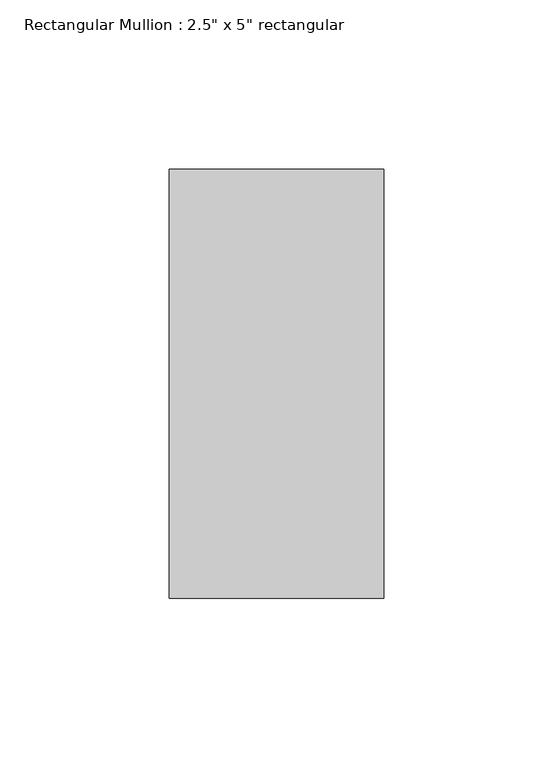
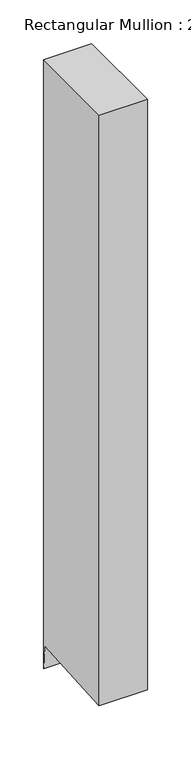
"""IFC4 building model written with IfcOpenShell, lengths in millimetres: member geometry."""

from ifc_helpers import new_model, si_unit, frame, origin, place, context, project, spatial, polyline, outline, extrude, source, transform, mapped, element, save


def member_bfce15ef(model_context):
    return source(origin(), model_context, "Body", "SweptSolid", [
        extrude(outline(polyline([(-63.5, 0.0), (63.5, 0.0), (63.5, -848.9346233), (61.4149606, -815.2837802), (-63.5, -823.0236342), (-63.5, 0.0)])), frame((-63.5, 0.0, 0.0), z_axis=(1.0, 0.0, 0.0), x_axis=(0.0, 1.0, 0.0)), (0.0, 0.0, 1.0), 63.5),
    ])


if __name__ == "__main__":
    model = new_model("IFC4")
    model_context = context("Model", 3, world=origin())
    ifc_project = project(units=[si_unit("LENGTHUNIT", "METRE", prefix="MILLI")], contexts=[model_context])
    site = spatial("IfcSite", under=ifc_project)
    building = spatial("IfcBuilding", under=site)
    placement = place(None, origin())
    member_shape = member_bfce15ef(model_context)
    element("IfcMember", 1, ObjectType="Rectangular Mullion : 2.5\" x 5\" rectangular", at=placement, inside=building, context=model_context, shape_type="MappedRepresentation", body=[
        mapped(member_shape, transform((0.0, 0.0, 0.0), x_axis=(1.0, 0.0, 0.0), y_axis=(0.0, 1.0, 0.0), z_axis=(0.0, 0.0, 1.0))),
    ])
    save(model, "model.ifc")

# Revit data of these elements
# Type "Rectangular Mullion : 2.5\" x 5\" rectangular"
#   built-in parameter 1007304 = 0.416667 (stored number, unit not read)
#   built-in parameter 1007301 = 0.104167 (stored number, unit not read)
#   built-in parameter 1007300 = 0.104167 (stored number, unit not read)
# Element 1 (IfcMember, "Rectangular Mullion : 2.5\" x 5\" rectangular")
#   Materials on its faces: "Metal - Aluminum"
# Materials
#   "Metal - Aluminum": class "Metal", colour RGB 247 247 247, transparency 0, Cost = 0
